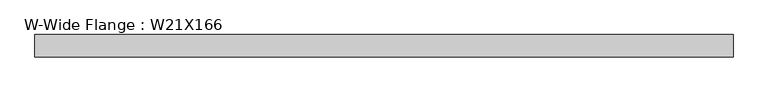
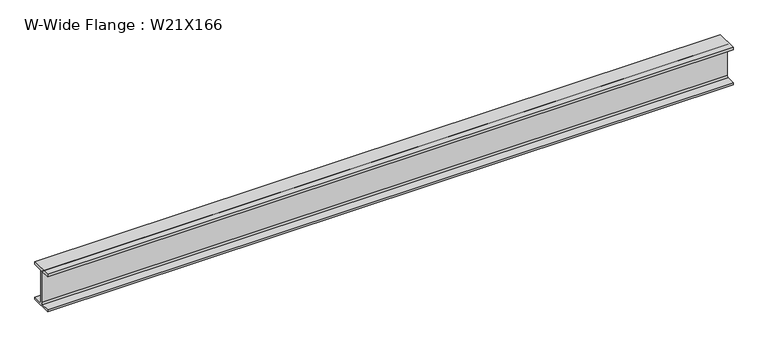
"""IFC4 building model written with IfcOpenShell, lengths in millimetres: beam geometry, W-Wide Flange : W21X166."""

from ifc_helpers import new_model, si_unit, point, frame, frame_2d, origin, place, context, project, spatial, polyline, circle_curve, trimmed, segment, composite_curve, outline, extrude, source, transform, mapped, element, save


def w_wide_flange_w21x166_1b8c9151(model_context):
    return source(origin(), model_context, "Body", "SweptSolid", [
        extrude(outline(composite_curve([segment(polyline([(157.48, -251.206), (157.48, -285.75), (-157.48, -285.75), (-157.48, -251.206), (-32.131, -251.206)]), True, "CONTINUOUS"), segment(trimmed(circle_curve(frame_2d((-32.131, -228.6)), 22.606), [point((-32.131, -251.206))], [point((-9.525, -228.6))], True, "CARTESIAN"), True, "CONTINUOUS"), segment(polyline([(-9.525, -228.6), (-9.525, 228.6)]), True, "CONTINUOUS"), segment(trimmed(circle_curve(frame_2d((-32.131, 228.6)), 22.606), [point((-9.525, 228.6))], [point((-32.131, 251.206))], True, "CARTESIAN"), True, "CONTINUOUS"), segment(polyline([(-32.131, 251.206), (-157.48, 251.206), (-157.48, 285.75), (157.48, 285.75), (157.48, 251.206), (32.131, 251.206)]), True, "CONTINUOUS"), segment(trimmed(circle_curve(frame_2d((32.131, 228.6)), 22.606), [point((32.131, 251.206))], [point((9.525, 228.6))], True, "CARTESIAN"), True, "CONTINUOUS"), segment(polyline([(9.525, 228.6), (9.525, -228.6)]), True, "CONTINUOUS"), segment(trimmed(circle_curve(frame_2d((32.131, -228.6)), 22.606), [point((9.525, -228.6))], [point((32.131, -251.206))], True, "CARTESIAN"), True, "CONTINUOUS"), segment(polyline([(32.131, -251.206), (157.48, -251.206)]), True, "CONTINUOUS")], self_intersect=False)), frame((-4963.0833359, 0.0, 0.0), z_axis=(1.0, 0.0, 0.0), x_axis=(0.0, 1.0, 0.0)), (0.0, 0.0, 1.0), 9898.83138),
    ])


if __name__ == "__main__":
    model = new_model("IFC4")
    model_context = context("Model", 3, world=origin())
    ifc_project = project(units=[si_unit("LENGTHUNIT", "METRE", prefix="MILLI")], contexts=[model_context])
    site = spatial("IfcSite", under=ifc_project)
    building = spatial("IfcBuilding", under=site)
    placement = place(None, origin())
    w_wide_flange_w21x166_shape = w_wide_flange_w21x166_1b8c9151(model_context)
    element("IfcBeam", 1, ObjectType="W-Wide Flange : W21X166", at=placement, inside=building, context=model_context, shape_type="MappedRepresentation", body=[
        mapped(w_wide_flange_w21x166_shape, transform((0.0, 0.0, 0.0), x_axis=(1.0, 0.0, 0.0), y_axis=(0.0, 1.0, 0.0), z_axis=(0.0, 0.0, 1.0))),
    ])
    save(model, "model.ifc")

# Revit data of these elements
# Type "W-Wide Flange : W21X166"
#   Assembly Code = "B10"
#   W = 166
#   Length [instance default] = 5' - 0"
#   bf = 1' - 0.4"
#   d = 1' - 10 1/2"
#   k = 0' - 2 1/4"
#   k2 = 0' - 0.89"
#   tf = 0' - 1.36"
#   tw = 0' - 0 3/4"
#   A = 0.338889 SF
#   Structural Material [instance default] = Steel ASTM A992
# Element 1 (IfcBeam, "W-Wide Flange : W21X166")
#   Materials on its faces: "Steel ASTM A992"
# Materials
#   "Steel ASTM A992": class "Metal", colour RGB 199 199 199, transparency 0, Description = "Structural steel 50ksi", Cost = 0
